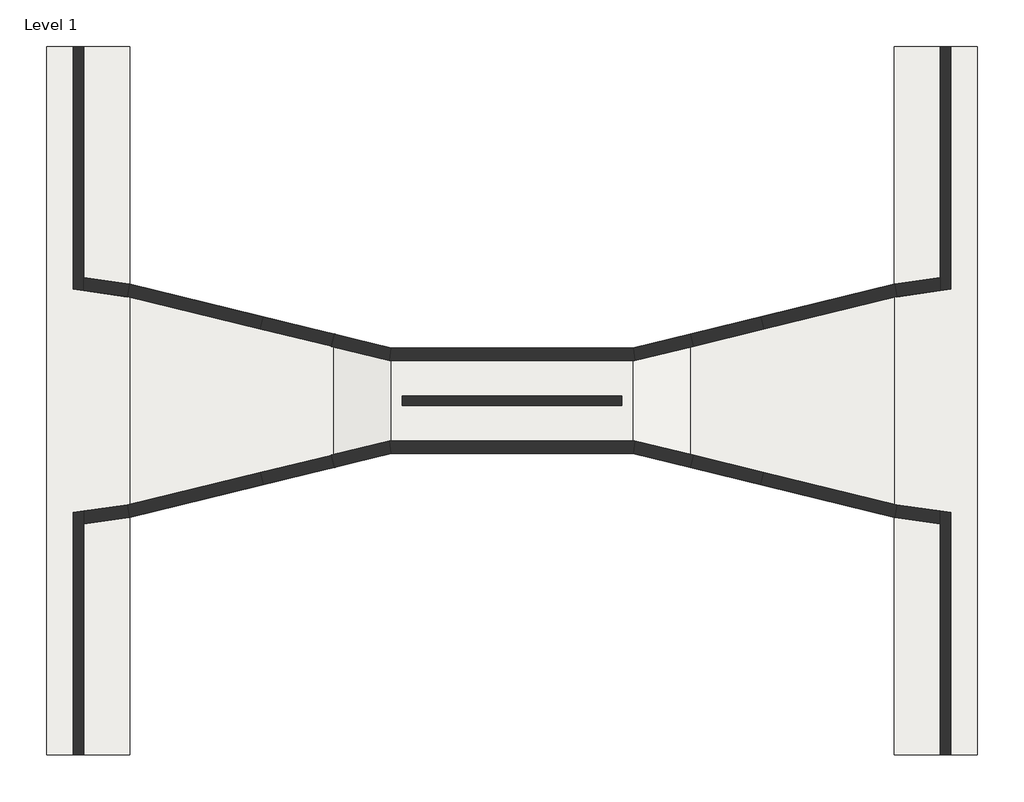
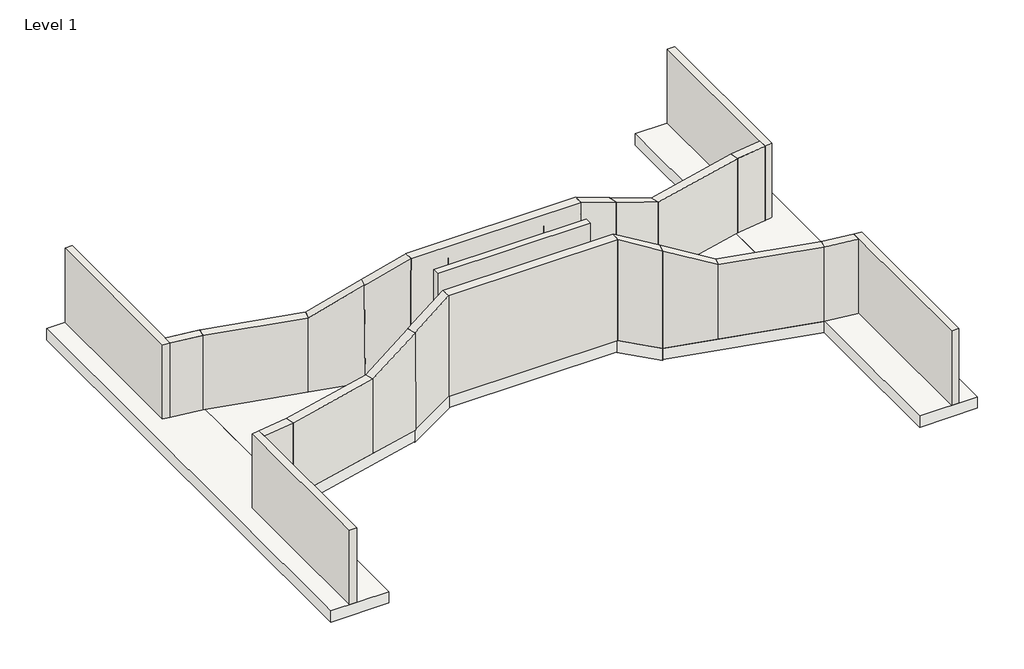
# One storey: 32 walls, 7 slabs.
"""IFC4 building model written with IfcOpenShell, lengths in millimetres."""

from ifc_helpers import new_model, si_unit, frame, origin, place, context, project, spatial, polyline, outline, extrude, faceted_brep, element, save

model = new_model("IFC4")

# Units and contexts
model_context = context("Model", 3, world=origin())
ifc_project = project(units=[si_unit("LENGTHUNIT", "METRE", prefix="MILLI")], contexts=[model_context])

# Site, building, storey
site = spatial("IfcSite", under=ifc_project)
building = spatial("IfcBuilding", under=site)
storey = spatial("IfcBuildingStorey", under=building, Name="Level 1", Elevation=0.0)

# Slabs
placement = place(None, origin())
element("IfcSlab", 1, ObjectType="Appronl", at=placement, inside=storey, context=model_context, shape_type="SweptSolid", body=[
    extrude(outline(polyline([(21800.0, -16601.0), (17901.0, -16601.0), (17901.0, 16601.0), (21800.0, 16601.0), (21800.0, -16601.0)])), frame((0.0, 0.0, -3600.0), z_axis=(0.0, 0.0, 1.0), x_axis=(1.0, 0.0, 0.0)), (0.0, 0.0, 1.0), 800.0),
])
element("IfcSlab", 2, ObjectType="Appronl", at=placement, inside=storey, context=model_context, shape_type="SweptSolid", body=[
    extrude(outline(polyline([(8350.0, 3127.0), (17901.0, 5458.0), (17901.0, -5458.0), (8350.0, -3127.0), (8350.0, 3127.0)])), frame((0.0, 0.0, -3600.0), z_axis=(0.0, 0.0, 1.0), x_axis=(1.0, 0.0, 0.0)), (0.0, 0.0, 1.0), 800.0),
])
element("IfcSlab", 3, ObjectType="Appronl", at=placement, inside=storey, context=model_context, shape_type="SweptSolid", body=[
    extrude(outline(polyline([(-21800.0, 16601.0), (-17901.0, 16601.0), (-17901.0, -16601.0), (-21800.0, -16601.0), (-21800.0, 16601.0)])), frame((0.0, 0.0, -3600.0), z_axis=(0.0, 0.0, 1.0), x_axis=(1.0, 0.0, 0.0)), (0.0, 0.0, 1.0), 800.0),
])
element("IfcSlab", 4, ObjectType="Appronl", at=placement, inside=storey, context=model_context, shape_type="SweptSolid", body=[
    extrude(outline(polyline([(-8350.0, 3127.0), (-8350.0, -3127.0), (-17901.0, -5458.0), (-17901.0, 5458.0), (-8350.0, 3127.0)])), frame((0.0, 0.0, -3600.0), z_axis=(0.0, 0.0, 1.0), x_axis=(1.0, 0.0, 0.0)), (0.0, 0.0, 1.0), 800.0),
])
element("IfcSlab", 5, ObjectType="Appronl", at=placement, inside=storey, context=model_context, shape_type="Brep", body=[
    faceted_brep([(-5650.0, 2468.0, -2563.8447252), (-5650.0, -2468.0, -2563.8447252), (-8350.0, -3127.0, -3663.8447252), (-8350.0, 3127.0, -3663.8447252), (-5650.0, 2468.0, -1700.0), (-8350.0, 3127.0, -2800.0), (-8350.0, -3127.0, -2800.0), (-5650.0, -2468.0, -1700.0)], [[[0, 1, 2, 3]], [[4, 5, 6, 7]], [[1, 0, 4, 7]], [[2, 1, 7, 6]], [[3, 2, 6, 5]], [[0, 3, 5, 4]]]),
])
element("IfcSlab", 6, ObjectType="Appronl", at=placement, inside=storey, context=model_context, shape_type="SweptSolid", body=[
    extrude(outline(polyline([(5650.0, 2468.0), (5650.0, -2468.0), (-5650.0, -2468.0), (-5650.0, 2468.0), (5650.0, 2468.0)])), frame((0.0, 0.0, -2500.0), z_axis=(0.0, 0.0, 1.0), x_axis=(1.0, 0.0, 0.0)), (0.0, 0.0, 1.0), 800.0),
])
element("IfcSlab", 7, ObjectType="Appronl", at=placement, inside=storey, context=model_context, shape_type="Brep", body=[
    faceted_brep([(5650.0, 2468.0, -2563.8447252), (8350.0, 3127.0, -3663.8447252), (8350.0, -3127.0, -3663.8447252), (5650.0, -2468.0, -2563.8447252), (5650.0, 2468.0, -1700.0), (5650.0, -2468.0, -1700.0), (8350.0, -3127.0, -2800.0), (8350.0, 3127.0, -2800.0)], [[[0, 1, 2, 3]], [[4, 5, 6, 7]], [[1, 0, 4, 7]], [[2, 1, 7, 6]], [[3, 2, 6, 5]], [[0, 3, 5, 4]]]),
])

# Walls
element("IfcWall", 8, ObjectType="Wingwall", at=placement, inside=storey, context=model_context, shape_type="SweptSolid", body=[
    extrude(outline(polyline([(-20050.0, 5767.2805137), (-17916.0428831, 5461.9054729), (-18029.9571169, 4872.0945271), (-20050.0, 5161.1681326), (-20050.0, 5767.2805137)])), frame((0.0, 0.0, -2800.0), z_axis=(0.0, 0.0, 1.0), x_axis=(1.0, 0.0, 0.0)), (0.0, 0.0, 1.0), 5300.0),
])
element("IfcWall", 9, ObjectType="Wingwall", at=placement, inside=storey, context=model_context, shape_type="SweptSolid", body=[
    extrude(outline(polyline([(-11792.4456337, 3349.3873565), (-18029.9571169, 4872.0945271), (-17916.0428831, 5461.9054729), (-11651.5543663, 3932.6126435), (-11792.4456337, 3349.3873565)])), frame((0.0, 0.0, -2800.0), z_axis=(0.0, 0.0, 1.0), x_axis=(1.0, 0.0, 0.0)), (0.0, 0.0, 1.0), 5300.0),
])
element("IfcWall", 10, ObjectType="Wingwall", at=placement, inside=storey, context=model_context, shape_type="Brep", body=[
    faceted_brep([(-11651.5543663, 3932.6126435, -2800.0), (-11651.5543663, 3932.6126435, 2500.3510698), (-8352.2565059, 3143.9904385, 4150.0), (-8280.2565059, 3126.780474, -2800.0), (-11792.4456336, 3349.3873565, -2800.0), (-8419.7434941, 2543.219526, -2800.0), (-8491.7434941, 2560.4294904, 4150.0), (-11792.4456336, 3349.3873565, 2499.6489302)], [[[0, 1, 2, 3]], [[4, 5, 6, 7]], [[2, 1, 7, 6]], [[3, 2, 6, 5]], [[0, 3, 5, 4]], [[1, 0, 4, 7]]]),
])
element("IfcWall", 11, ObjectType="Wingwall", at=placement, inside=storey, context=model_context, shape_type="Brep", body=[
    faceted_brep([(-8350.8659334, 3126.4445823, 4150.0), (-5685.9184792, 2476.0, 5482.4737271), (-5685.9184792, 2476.0, -1714.671918), (-8278.8659334, 3108.871249, -2800.0), (-8493.1340666, 2543.5554177, 4150.0), (-8421.1340666, 2525.9820843, -2800.0), (-5758.0815208, 1876.0, -1685.328082), (-5758.0815208, 1876.0, 5517.5262729)], [[[0, 1, 2, 3]], [[4, 5, 6, 7]], [[1, 0, 4, 7]], [[3, 2, 6, 5]], [[0, 3, 5, 4]], [[1, 7, 6, 2]]]),
])
element("IfcWall", 12, ObjectType="Wingwall", at=placement, inside=storey, context=model_context, shape_type="Brep", body=[
    faceted_brep([(5685.9184792, 2476.0, -1714.2806668), (5685.9184792, 2476.0, 5482.4737271), (8350.8659334, 3126.4445823, 4150.0), (8350.8659334, 3126.4445823, -2800.0), (5758.0815208, 1876.0, 5517.5262729), (5758.0815208, 1876.0, -1685.7193332), (8493.1340666, 2543.5554177, -2800.0), (8493.1340666, 2543.5554177, 4150.0)], [[[0, 1, 2, 3]], [[4, 5, 6, 7]], [[2, 1, 4, 7]], [[0, 3, 6, 5]], [[2, 7, 6, 3]], [[0, 5, 4, 1]]]),
])
element("IfcWall", 13, ObjectType="Wingwall", at=placement, inside=storey, context=model_context, shape_type="SweptSolid", body=[
    extrude(outline(polyline([(18029.9571169, 4872.0945271), (11793.1469574, 3349.5585643), (11650.8530426, 3932.4414357), (17916.0428831, 5461.9054729), (18029.9571169, 4872.0945271)])), frame((0.0, 0.0, -2800.0), z_axis=(0.0, 0.0, 1.0), x_axis=(1.0, 0.0, 0.0)), (0.0, 0.0, 1.0), 5300.0),
])
element("IfcWall", 14, ObjectType="Wingwall", at=placement, inside=storey, context=model_context, shape_type="SweptSolid", body=[
    extrude(outline(polyline([(17916.0428831, 5461.9054729), (20050.0, 5767.2805137), (20050.0, 5161.1681326), (18029.9571169, 4872.0945271), (17916.0428831, 5461.9054729)])), frame((0.0, 0.0, -2800.0), z_axis=(0.0, 0.0, 1.0), x_axis=(1.0, 0.0, 0.0)), (0.0, 0.0, 1.0), 5300.0),
])
element("IfcWall", 15, ObjectType="Wingwall", at=placement, inside=storey, context=model_context, shape_type="SweptSolid", body=[
    extrude(outline(polyline([(5300.0, 0.0), (6950.0, -3397.0039741), (0.0, -3397.0039741), (0.0, 0.0), (5300.0, 0.0)])), frame((11793.1803701, 3349.566723, -2800.0), z_axis=(-0.23726790022826785, 0.9714442565177216, 0.0), x_axis=(0.0, 0.0, 1.0)), (0.0, 0.0, 1.0), 600.0),
])
element("IfcWall", 16, ObjectType="Wingwall", at=placement, inside=storey, context=model_context, shape_type="SweptSolid", body=[
    extrude(outline(polyline([(-20050.0, -5161.1681326), (-18029.9571169, -4872.0945271), (-17916.0428831, -5461.9054729), (-20050.0, -5767.2805137), (-20050.0, -5161.1681326)])), frame((0.0, 0.0, -2800.0), z_axis=(0.0, 0.0, 1.0), x_axis=(1.0, 0.0, 0.0)), (0.0, 0.0, 1.0), 5300.0),
])
element("IfcWall", 17, ObjectType="Wingwall", at=placement, inside=storey, context=model_context, shape_type="SweptSolid", body=[
    extrude(outline(polyline([(-11651.5543663, -3932.6126435), (-17916.0428831, -5461.9054729), (-18029.9571169, -4872.0945271), (-11792.4456337, -3349.3873565), (-11651.5543663, -3932.6126435)])), frame((0.0, 0.0, -2800.0), z_axis=(0.0, 0.0, 1.0), x_axis=(1.0, 0.0, 0.0)), (0.0, 0.0, 1.0), 5300.0),
])
element("IfcWall", 18, ObjectType="Wingwall", at=placement, inside=storey, context=model_context, shape_type="Brep", body=[
    faceted_brep([(-11792.4456336, -3349.3873565, -2800.0), (-11792.4456336, -3349.3873565, 2499.6489302), (-8491.7434941, -2560.4294904, 4150.0), (-8419.7434941, -2543.219526, -2800.0), (-11651.5543663, -3932.6126435, -2800.0), (-8280.2565059, -3126.780474, -2800.0), (-8352.2565059, -3143.9904385, 4150.0), (-11651.5543663, -3932.6126435, 2500.3510698)], [[[0, 1, 2, 3]], [[4, 5, 6, 7]], [[2, 1, 7, 6]], [[3, 2, 6, 5]], [[0, 3, 5, 4]], [[1, 0, 4, 7]]]),
])
element("IfcWall", 19, ObjectType="Wingwall", at=placement, inside=storey, context=model_context, shape_type="Brep", body=[
    faceted_brep([(-8493.1340666, -2543.5554177, 4150.0), (-5758.0815208, -1876.0, 5517.5262729), (-5758.0815208, -1876.0, -1685.328082), (-8421.1340666, -2525.9820843, -2800.0), (-8350.8659334, -3126.4445823, 4150.0), (-8278.8659334, -3108.871249, -2800.0), (-5685.9184792, -2476.0, -1714.671918), (-5685.9184792, -2476.0, 5482.4737271)], [[[0, 1, 2, 3]], [[4, 5, 6, 7]], [[1, 0, 4, 7]], [[3, 2, 6, 5]], [[0, 3, 5, 4]], [[2, 1, 7, 6]]]),
])
element("IfcWall", 20, ObjectType="Wingwall", at=placement, inside=storey, context=model_context, shape_type="Brep", body=[
    faceted_brep([(5758.0815208, -1876.0, -1685.7193332), (5758.0815208, -1876.0, 5517.5262729), (8493.1340666, -2543.5554177, 4150.0), (8493.1340666, -2543.5554177, -2800.0), (5685.9184792, -2476.0, -1714.2806668), (8350.8659334, -3126.4445823, -2800.0), (8350.8659334, -3126.4445823, 4150.0), (5685.9184792, -2476.0, 5482.4737271)], [[[0, 1, 2, 3]], [[4, 5, 6, 7]], [[2, 1, 7, 6]], [[3, 2, 6, 5]], [[0, 3, 5, 4]], [[1, 0, 4, 7]]]),
])
element("IfcWall", 21, ObjectType="Wingwall", at=placement, inside=storey, context=model_context, shape_type="SweptSolid", body=[
    extrude(outline(polyline([(5300.0, 0.0), (6950.0, -3397.0039741), (0.0, -3397.0039741), (0.0, 0.0), (5300.0, 0.0)])), frame((11650.8196299, -3932.433277, -2800.0), z_axis=(0.23726790022826785, 0.9714442565177216, 0.0), x_axis=(0.0, 0.0, 1.0)), (0.0, 0.0, 1.0), 600.0),
])
element("IfcWall", 22, ObjectType="Wingwall", at=placement, inside=storey, context=model_context, shape_type="SweptSolid", body=[
    extrude(outline(polyline([(17916.0428831, -5461.9054729), (11650.8530426, -3932.4414357), (11793.1469574, -3349.5585643), (18029.9571169, -4872.0945271), (17916.0428831, -5461.9054729)])), frame((0.0, 0.0, -2800.0), z_axis=(0.0, 0.0, 1.0), x_axis=(1.0, 0.0, 0.0)), (0.0, 0.0, 1.0), 5300.0),
])
element("IfcWall", 23, ObjectType="Wingwall", at=placement, inside=storey, context=model_context, shape_type="SweptSolid", body=[
    extrude(outline(polyline([(18029.9571169, -4872.0945271), (20050.0, -5161.1681326), (20050.0, -5767.2805137), (17916.0428831, -5461.9054729), (18029.9571169, -4872.0945271)])), frame((0.0, 0.0, -2800.0), z_axis=(0.0, 0.0, 1.0), x_axis=(1.0, 0.0, 0.0)), (0.0, 0.0, 1.0), 5300.0),
])
element("IfcWall", 24, ObjectType="Wingwall", at=placement, inside=storey, context=model_context, shape_type="SweptSolid", body=[
    extrude(outline(polyline([(-20050.0, 5767.2805137), (-17930.5021265, 5463.9746298), (-18015.4978735, 4870.0253702), (-20050.0, 5161.1681326), (-20050.0, 5767.2805137)])), frame((0.0, 0.0, -2800.0), z_axis=(0.0, 0.0, 1.0), x_axis=(1.0, 0.0, 0.0)), (0.0, 0.0, 1.0), 5300.0),
])
element("IfcWall", 25, ObjectType="Wingwall", at=placement, inside=storey, context=model_context, shape_type="SweptSolid", body=[
    extrude(outline(polyline([(-11793.1469574, 3349.5585643), (-18029.9571169, 4872.0945271), (-17916.0428831, 5461.9054729), (-11650.8530426, 3932.4414357), (-11793.1469574, 3349.5585643)])), frame((0.0, 0.0, -2800.0), z_axis=(0.0, 0.0, 1.0), x_axis=(1.0, 0.0, 0.0)), (0.0, 0.0, 1.0), 5300.0),
])
element("IfcWall", 26, ObjectType="Wingwall", at=placement, inside=storey, context=model_context, shape_type="Brep", body=[
    faceted_brep([(-11651.5543663, 3932.6126435, -2800.0), (-11651.5543663, 3932.6126435, 2500.3510698), (-8352.2565059, 3143.9904385, 4150.0), (-8280.2565059, 3126.780474, -2800.0), (-11792.4456336, 3349.3873565, -2800.0), (-8419.7434941, 2543.219526, -2800.0), (-8491.7434941, 2560.4294904, 4150.0), (-11792.4456336, 3349.3873565, 2499.6489302)], [[[0, 1, 2, 3]], [[4, 5, 6, 7]], [[2, 1, 7, 6]], [[3, 2, 6, 5]], [[0, 3, 5, 4]], [[1, 0, 4, 7]]]),
])
element("IfcWall", 27, ObjectType="Wingwall", at=placement, inside=storey, context=model_context, shape_type="Brep", body=[
    faceted_brep([(-8350.8659334, 3126.4445823, 4150.0), (-5685.9184792, 2476.0, 5482.4737271), (-5685.9184792, 2476.0, -1714.671918), (-8278.8659334, 3108.871249, -2800.0), (-8493.1340666, 2543.5554177, 4150.0), (-8421.1340666, 2525.9820843, -2800.0), (-5758.0815208, 1876.0, -1685.328082), (-5758.0815208, 1876.0, 5517.5262729)], [[[0, 1, 2, 3]], [[4, 5, 6, 7]], [[1, 0, 4, 7]], [[3, 2, 6, 5]], [[0, 3, 5, 4]], [[1, 7, 6, 2]]]),
])
element("IfcWall", 28, ObjectType="Wingwall", at=placement, inside=storey, context=model_context, shape_type="Brep", body=[
    faceted_brep([(5685.9184792, 2476.0, -1714.2806668), (5685.9184792, 2476.0, 5482.4737271), (8350.8659334, 3126.4445823, 4150.0), (8350.8659334, 3126.4445823, -2800.0), (5758.0815208, 1876.0, 5517.5262729), (5758.0815208, 1876.0, -1685.7193332), (8493.1340666, 2543.5554177, -2800.0), (8493.1340666, 2543.5554177, 4150.0)], [[[0, 1, 2, 3]], [[4, 5, 6, 7]], [[2, 1, 4, 7]], [[0, 3, 6, 5]], [[0, 5, 4, 1]], [[2, 7, 6, 3]]]),
])
element("IfcWall", 29, ObjectType="Wingwall", at=placement, inside=storey, context=model_context, shape_type="SweptSolid", body=[
    extrude(outline(polyline([(5300.0, 0.0), (6950.0, -3397.0039741), (0.0, -3397.0039741), (0.0, 0.0), (5300.0, 0.0)])), frame((11793.1803701, 3349.566723, -2800.0), z_axis=(-0.23726790022826785, 0.9714442565177216, 0.0), x_axis=(0.0, 0.0, 1.0)), (0.0, 0.0, 1.0), 600.0),
])
element("IfcWall", 30, ObjectType="Wingwall", at=placement, inside=storey, context=model_context, shape_type="SweptSolid", body=[
    extrude(outline(polyline([(18029.9571169, 4872.0945271), (11793.1469574, 3349.5585643), (11650.8530426, 3932.4414357), (17916.0428831, 5461.9054729), (18029.9571169, 4872.0945271)])), frame((0.0, 0.0, -2800.0), z_axis=(0.0, 0.0, 1.0), x_axis=(1.0, 0.0, 0.0)), (0.0, 0.0, 1.0), 5300.0),
])
element("IfcWall", 31, ObjectType="Wingwall", at=placement, inside=storey, context=model_context, shape_type="SweptSolid", body=[
    extrude(outline(polyline([(17930.5021265, 5463.9746298), (20050.0, 5767.2805137), (20050.0, 5161.1681326), (18015.4978735, 4870.0253702), (17930.5021265, 5463.9746298)])), frame((0.0, 0.0, -2800.0), z_axis=(0.0, 0.0, 1.0), x_axis=(1.0, 0.0, 0.0)), (0.0, 0.0, 1.0), 5300.0),
])
element("IfcWall", 32, ObjectType="Abutment", at=placement, inside=storey, context=model_context, shape_type="Brep", body=[
    faceted_brep([(-5758.0815208, 1876.0, -1700.0), (5758.0815208, 1876.0, -1700.0), (5758.0815208, 1876.0, 4673.4903305), (5722.0, 1876.0, 4673.4903305), (5722.0, 1876.0, 5500.0), (-5722.0, 1876.0, 5500.0), (-5722.0, 1876.0, 4673.4903305), (-5758.0815208, 1876.0, 4673.4903305), (-5685.9184792, 2476.0, -1700.0), (-5685.9184792, 2476.0, 4673.4903305), (-5722.0, 2476.0, 4673.4903305), (-5722.0, 2476.0, 5500.0), (5722.0, 2476.0, 5500.0), (5722.0, 2476.0, 4673.4903305), (5685.9184792, 2476.0, 4673.4903305), (5685.9184792, 2476.0, -1700.0), (-5722.0, 2176.0, 4673.4903305), (5722.0, 2176.0, 4673.4903305)], [[[0, 1, 2, 3, 4, 5, 6, 7]], [[8, 9, 10, 11, 12, 13, 14, 15]], [[1, 0, 8, 15]], [[5, 4, 12, 11]], [[6, 5, 11, 10, 16]], [[6, 16, 7]], [[0, 7, 16, 9, 8]], [[16, 10, 9]], [[4, 3, 17, 13, 12]], [[13, 17, 14]], [[2, 1, 15, 14, 17]], [[17, 3, 2]]]),
])
element("IfcWall", 33, ObjectType="Abutment", at=placement, inside=storey, context=model_context, shape_type="SweptSolid", body=[
    extrude(outline(polyline([(5685.9184792, -2476.0), (-5685.9184792, -2476.0), (-5758.0815208, -1876.0), (5758.0815208, -1876.0), (5685.9184792, -2476.0)])), frame((0.0, 0.0, -1700.0), z_axis=(0.0, 0.0, 1.0), x_axis=(1.0, 0.0, 0.0)), (0.0, 0.0, 1.0), 7200.0),
])
element("IfcWall", 34, ObjectType="Abutment", at=placement, inside=storey, context=model_context, shape_type="Brep", body=[
    faceted_brep([(-3227.648373, 1876.0, -1700.0), (3227.648373, 1876.0, -1700.0), (3227.648373, 1876.0, 4673.4903305), (5722.0, 1876.0, 4673.4903305), (5722.0, 1876.0, 5500.0), (-5722.0, 1876.0, 5500.0), (-5722.0, 1876.0, 4673.4903305), (-3227.648373, 1876.0, 4673.4903305), (-5685.9184792, 2476.0, -1700.0), (-5685.9184792, 2476.0, 4673.4903305), (-5722.0, 2476.0, 4673.4903305), (-5722.0, 2476.0, 5500.0), (5722.0, 2476.0, 5500.0), (5722.0, 2476.0, 4673.4903305), (5685.9184792, 2476.0, 4673.4903305), (5685.9184792, 2476.0, -1700.0)], [[[0, 1, 2, 3, 4, 5, 6, 7]], [[8, 9, 10, 11, 12, 13, 14, 15]], [[1, 0, 8, 15]], [[5, 4, 12, 11]], [[6, 5, 11, 10]], [[6, 10, 9, 7]], [[0, 7, 9, 8]], [[4, 3, 13, 12]], [[13, 3, 2, 14]], [[2, 1, 15, 14]]]),
])
element("IfcWall", 35, ObjectType="Pier", at=placement, inside=storey, context=model_context, shape_type="SweptSolid", body=[
    extrude(outline(polyline([(5150.0, -225.0), (-5150.0, -225.0), (-5150.0, 225.0), (5150.0, 225.0), (5150.0, -225.0)])), frame((0.0, 0.0, -1700.0), z_axis=(0.0, 0.0, 1.0), x_axis=(1.0, 0.0, 0.0)), (0.0, 0.0, 1.0), 7200.0),
])
element("IfcWall", 36, ObjectType="Return Wall", at=placement, inside=storey, context=model_context, shape_type="Brep", body=[
    faceted_brep([(20550.0, 5232.7194863, -2800.0), (20550.0, 16601.0, -2800.0), (20550.0, 16601.0, 2500.0), (20550.0, 5232.7194863, 2500.0), (20050.0, 5161.1681326, -2800.0), (20050.0, 5161.1681326, 2500.0), (20050.0, 5767.2805137, 2500.0), (20050.0, 16601.0, 2500.0), (20050.0, 16601.0, -2800.0), (20050.0, 5767.2805137, -2800.0)], [[[0, 1, 2, 3]], [[4, 5, 6, 7, 8, 9]], [[1, 0, 4, 9, 8]], [[2, 1, 8, 7]], [[3, 2, 7, 6, 5]], [[0, 3, 5, 4]]]),
])
element("IfcWall", 37, ObjectType="Return Wall", at=placement, inside=storey, context=model_context, shape_type="Brep", body=[
    faceted_brep([(20550.0, -16601.0, -2800.0), (20550.0, -5232.7194863, -2800.0), (20550.0, -5232.7194863, 2500.0), (20550.0, -16601.0, 2500.0), (20050.0, -16601.0, -2800.0), (20050.0, -16601.0, 2500.0), (20050.0, -5767.2805137, 2500.0), (20050.0, -5161.1681326, 2500.0), (20050.0, -5161.1681326, -2800.0), (20050.0, -5767.2805137, -2800.0)], [[[0, 1, 2, 3]], [[4, 5, 6, 7, 8, 9]], [[1, 0, 4, 9, 8]], [[3, 2, 7, 6, 5]], [[0, 3, 5, 4]], [[2, 1, 8, 7]]]),
])
element("IfcWall", 38, ObjectType="Return Wall", at=placement, inside=storey, context=model_context, shape_type="Brep", body=[
    faceted_brep([(-20050.0, -16601.0, -2800.0), (-20050.0, -5767.2805137, -2800.0), (-20050.0, -5161.1681326, -2800.0), (-20050.0, -5161.1681326, 2500.0), (-20050.0, -5767.2805137, 2500.0), (-20050.0, -16601.0, 2500.0), (-20550.0, -16601.0, -2800.0), (-20550.0, -16601.0, 2500.0), (-20550.0, -5232.7194863, 2500.0), (-20550.0, -5232.7194863, -2800.0)], [[[0, 1, 2, 3, 4, 5]], [[6, 7, 8, 9]], [[2, 1, 0, 6, 9]], [[5, 4, 3, 8, 7]], [[0, 5, 7, 6]], [[3, 2, 9, 8]]]),
])
element("IfcWall", 39, ObjectType="Return Wall", at=placement, inside=storey, context=model_context, shape_type="Brep", body=[
    faceted_brep([(-20050.0, 5161.1681326, -2800.0), (-20050.0, 5767.2805137, -2800.0), (-20050.0, 16601.0, -2800.0), (-20050.0, 16601.0, 2500.0), (-20050.0, 5767.2805137, 2500.0), (-20050.0, 5161.1681326, 2500.0), (-20550.0, 5232.7194863, -2800.0), (-20550.0, 5232.7194863, 2500.0), (-20550.0, 16601.0, 2500.0), (-20550.0, 16601.0, -2800.0)], [[[0, 1, 2, 3, 4, 5]], [[6, 7, 8, 9]], [[2, 1, 0, 6, 9]], [[3, 2, 9, 8]], [[5, 4, 3, 8, 7]], [[0, 5, 7, 6]]]),
])

save(model, "model.ifc")

# Revit data of these elements
# Project information
#   Project Issue Date = "Issue Date"
#   Project Status = "Project Status"
#   Client Name = "Owner"
#   Project Address = "Enter address here"
#   Project Name = "Project Name"
#   Project Number = "Project Number"
# Type "Appronl"
#   Assembly Code = "B1010"
#   Function = 0
#   Layers, outside or top first: 800 mm "CONCR" (function 1)
# Type "Wingwall"
#   Assembly Code = "B2010"
#   Layers, outside or top first: 600 mm "CONCR" (function 1)
# Type "Abutment"
#   Assembly Code = "B2010"
#   Layers, outside or top first: 600 mm "CONCR" (function 1)
# Type "Pier"
#   Assembly Code = "B2010"
#   Layers, outside or top first: 450 mm "CONCR" (function 1)
# Type "Return Wall"
#   Assembly Code = "B2010"
#   Layers, outside or top first: 500 mm "CONCR" (function 1)
# Elements 1, 2, 3, 4, 5, 7 (IfcSlab, "Appronl")
#   Height Offset From Level = -2800 mm
#   built-in parameter 1001954 = 1
#   Phase Created = New Construction
#   Materials on its faces: "CONCR"
# Element 6 (IfcSlab, "Appronl")
#   Height Offset From Level = -1700 mm
#   built-in parameter 1001954 = 1
#   Phase Created = New Construction
#   Materials on its faces: "CONCR"
# Elements 8, 9, 13, 14, 16, 17, 22, 23, 24, 25, 30, 31 (IfcWall, "Wingwall")
#   built-in parameter 1001111 = -2800 mm
#   Top Offset = -548 mm
#   Base Offset = -2800 mm
#   Unconnected Height = 5300 mm
#   wall height = 5300 mm
#   Phase Created = New Construction
#   Base Constraint = Level 1
#   Top Constraint = Level 2
#   Materials on its faces: "CONCR"
# Elements 10, 15, 18, 21, 26, 29 (IfcWall, "Wingwall")
#   built-in parameter 1001111 = -2800 mm
#   Top Offset = 1102 mm
#   Base Offset = -2800 mm
#   Unconnected Height = 6950 mm
#   wall height = 6950 mm
#   Phase Created = New Construction
#   Base Constraint = Level 1
#   Top Constraint = Level 2
#   Materials on its faces: "CONCR"
# Elements 11, 12, 19, 20, 27, 28 (IfcWall, "Wingwall")
#   built-in parameter 1001111 = -2800 mm
#   Top Offset = 2452 mm
#   Base Offset = -2800 mm
#   Unconnected Height = 8300 mm
#   wall height = 8300 mm
#   Phase Created = New Construction
#   Base Constraint = Level 1
#   Top Constraint = Level 2
#   Materials on its faces: "CONCR"
# Elements 32, 33, 34 (IfcWall, "Abutment")
#   built-in parameter 1001111 = -1700 mm
#   Top Offset = 2452 mm
#   Base Offset = -1700 mm
#   Unconnected Height = 7200 mm
#   wall height = 7200 mm
#   Phase Created = New Construction
#   Base Constraint = Level 1
#   Top Constraint = Level 2
#   Materials on its faces: "CONCR"
# Element 35 (IfcWall, "Pier")
#   built-in parameter 1001111 = -1700 mm
#   Top Offset = 2452 mm
#   Base Offset = -1700 mm
#   Unconnected Height = 7200 mm
#   wall height = 7200 mm
#   Phase Created = New Construction
#   Base Constraint = Level 1
#   Top Constraint = Level 2
#   Materials on its faces: "CONCR"
# Elements 36, 37, 38, 39 (IfcWall, "Return Wall")
#   built-in parameter 1001111 = -2800 mm
#   Top Offset = -548 mm
#   Base Offset = -2800 mm
#   Unconnected Height = 5300 mm
#   wall height = 5300 mm
#   Phase Created = New Construction
#   Base Constraint = Level 1
#   Top Constraint = Level 2
#   Materials on its faces: "CONCR"
# Materials
#   "CONCR": class "Unassigned", colour RGB 192 192 192, transparency 0
